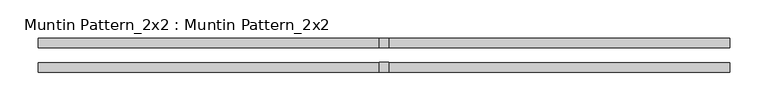
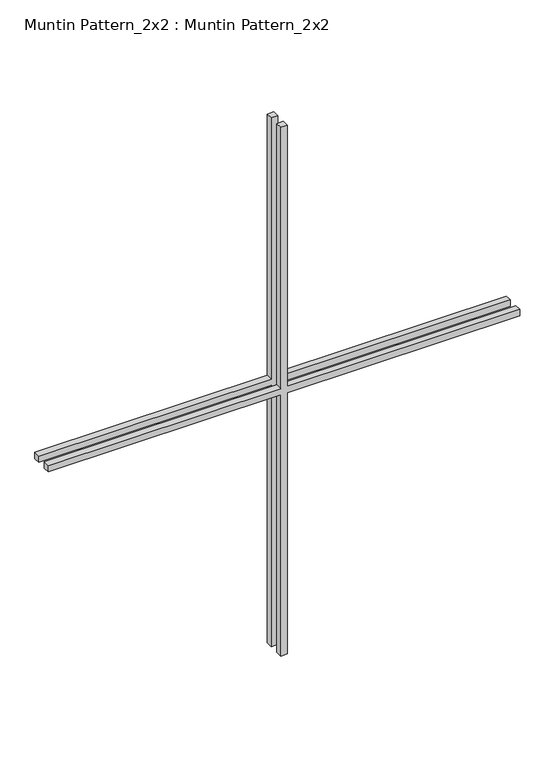
"""IFC4 building model written with IfcOpenShell, lengths in millimetres: proxy geometry, Muntin Pattern_2x2 : Muntin Pattern_2x2."""

from ifc_helpers import new_model, si_unit, frame, origin, place, context, project, spatial, polyline, outline, extrude, source, transform, mapped, element, save


def muntin_pattern_2x2_muntin_pattern_2x2_4e1ccfa3(model_context):
    return source(origin(), model_context, "Body", "SweptSolid", [
        extrude(outline(polyline([(542.925, -6.35), (542.925, -452.4375), (530.225, -452.4375), (530.225, -6.35), (0.0, -6.35), (0.0, 6.35), (530.225, 6.35), (530.225, 452.4375), (542.925, 452.4375), (542.925, 6.35), (1073.15, 6.35), (1073.15, -6.35), (542.925, -6.35)])), frame((0.0, 9.525, 0.0), z_axis=(0.0, 1.0, 0.0), x_axis=(0.0, 0.0, 1.0)), (0.0, 0.0, 1.0), 12.7),
        extrude(outline(polyline([(542.925, -6.35), (542.925, -452.4375), (530.225, -452.4375), (530.225, -6.35), (0.0, -6.35), (0.0, 6.35), (530.225, 6.35), (530.225, 452.4375), (542.925, 452.4375), (542.925, 6.35), (1073.15, 6.35), (1073.15, -6.35), (542.925, -6.35)])), frame((0.0, -22.225, 0.0), z_axis=(0.0, 1.0, 0.0), x_axis=(0.0, 0.0, 1.0)), (0.0, 0.0, 1.0), 12.7),
    ])


if __name__ == "__main__":
    model = new_model("IFC4")
    model_context = context("Model", 3, world=origin())
    ifc_project = project(units=[si_unit("LENGTHUNIT", "METRE", prefix="MILLI")], contexts=[model_context])
    site = spatial("IfcSite", under=ifc_project)
    building = spatial("IfcBuilding", under=site)
    placement = place(None, origin())
    muntin_pattern_2x2_muntin_pattern_2x2_shape = muntin_pattern_2x2_muntin_pattern_2x2_4e1ccfa3(model_context)
    element("IfcBuildingElementProxy", 1, Name="Muntin Pattern_2x2 : Muntin Pattern_2x2", ObjectType="Muntin Pattern_2x2 : Muntin Pattern_2x2", at=placement, inside=building, context=model_context, shape_type="MappedRepresentation", body=[
        mapped(muntin_pattern_2x2_muntin_pattern_2x2_shape, transform((0.0, 0.0, 0.0), x_axis=(1.0, 0.0, 0.0), y_axis=(0.0, 1.0, 0.0), z_axis=(0.0, 0.0, 1.0))),
    ])
    save(model, "model.ifc")

# Revit data of these elements
# Type "Muntin Pattern_2x2 : Muntin Pattern_2x2"
#   Width [instance default] = 4' - 0"
#   Thickness = 0' - 0 1/2"
#   Height [instance default] = 4' - 0"
#   Distance = 0' - 0 3/4"
#   Interior Material [instance default] = none
#   Exterior Material [instance default] = none
#   Default Elevation = 0
# Element 1 (IfcBuildingElementProxy, "Muntin Pattern_2x2 : Muntin Pattern_2x2")
#   Width = 2' - 11 5/8"
#   Height = 3' - 6 1/4"
#   Interior Material = Wood - Stained
#   Exterior Material = Clad - White
#   Materials on its faces: "Clad - White", "Wood - Stained"
# Materials
#   "Clad - White": class "Wood", colour RGB 242 242 238, transparency 0, Cost = 0
#   "Wood - Stained": class "Wood", colour RGB 224 178 126, transparency 0, Cost = 0
